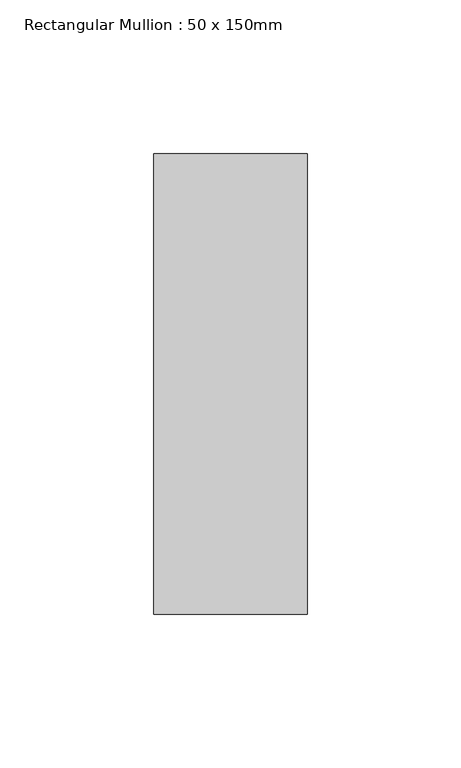
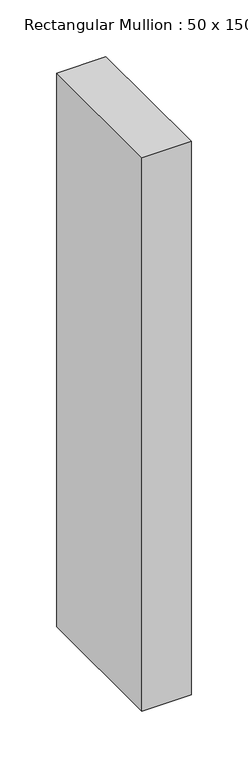
"""IFC4 building model written with IfcOpenShell, lengths in millimetres: member geometry, Rectangular Mullion : 50 x 150mm."""

import ifcopenshell
import ifcopenshell.guid

model = None  # the IFC model being written
_history = None  # IfcOwnerHistory: only IFC2X3 demands one
_inside = {}  # id of a spatial element -> (the spatial element, [elements in it])
_under = {}  # id of a project, library or spatial element -> (it, [spatial elements below it])
_declared = {}  # id of a project -> (the project, [libraries it declares])
_typed = {}  # id of a type object -> (the type object, [elements of that type])
_made_of = {}  # id of a material, layer set ... -> (it, [elements and type objects made of it])


def new_model(schema):
    """Start an empty IFC model of exactly this schema.

    Asked for "IFC4X3", IfcOpenShell would pick the latest addendum, in which some entities
    have other attributes; the version numbers below select the first issue.
    IFC2X3 requires an IfcOwnerHistory on every rooted entity: one is made here for all.
    """
    global model, _history
    if schema == "IFC4X3":
        model = ifcopenshell.file(schema_version=(4, 3, 0, 0))
    else:
        model = ifcopenshell.file(schema=schema)
    _inside.clear()
    _under.clear()
    _declared.clear()
    _typed.clear()
    _made_of.clear()
    _history = None
    if model.schema == "IFC2X3":
        org = make("IfcOrganization", Name="unknown")
        user = make(
            "IfcPersonAndOrganization",
            ThePerson=make("IfcPerson", FamilyName="unknown"),
            TheOrganization=org,
        )
        app = make(
            "IfcApplication",
            ApplicationDeveloper=org,
            Version="unknown",
            ApplicationFullName="unknown",
            ApplicationIdentifier="unknown",
        )
        _history = make(
            "IfcOwnerHistory",
            OwningUser=user,
            OwningApplication=app,
            ChangeAction="ADDED",
            CreationDate=0,
        )
    return model


def make(cls, **values):
    """One entity of the class cls with the attributes given. An attribute that is None is left unset."""
    return model.create_entity(
        cls, **{name: value for name, value in values.items() if value is not None}
    )


def rooted(cls, **values):
    """An entity with a GlobalId (a new one), such as an element, a storey or a relation."""
    return make(cls, GlobalId=ifcopenshell.guid.new(), OwnerHistory=_history, **values)


def si_unit(unit_type, name, prefix=None):
    """IfcSIUnit, for example si_unit("LENGTHUNIT", "METRE", prefix="MILLI")."""
    return make("IfcSIUnit", UnitType=unit_type, Prefix=prefix, Name=name)


def assignment(units):
    """IfcUnitAssignment: the units of a project."""
    return None if units is None else make("IfcUnitAssignment", Units=units)


def point(xyz):
    """IfcCartesianPoint."""
    return None if xyz is None else make("IfcCartesianPoint", Coordinates=xyz)


def direction(xyz):
    """IfcDirection."""
    return None if xyz is None else make("IfcDirection", DirectionRatios=xyz)


def frame(location, z_axis=None, x_axis=None):
    """IfcAxis2Placement3D, a coordinate frame: its origin and axes. An axis left out is left unset."""
    return make(
        "IfcAxis2Placement3D",
        Location=point(location),
        Axis=direction(z_axis),
        RefDirection=direction(x_axis),
    )


def origin():
    """The frame at (0, 0, 0) with its axes left unset."""
    return frame((0.0, 0.0, 0.0))


def place(relative_to, where):
    """IfcLocalPlacement: puts the frame where relative to a parent placement (None: the world)."""
    return make(
        "IfcLocalPlacement", PlacementRelTo=relative_to, RelativePlacement=where
    )


def context(
    kind, dimensions, precision=None, world=None, true_north=None, identifier=None
):
    """IfcGeometricRepresentationContext, for example the 3D "Model" context."""
    return make(
        "IfcGeometricRepresentationContext",
        ContextIdentifier=identifier,
        ContextType=kind,
        CoordinateSpaceDimension=dimensions,
        Precision=precision,
        WorldCoordinateSystem=world,
        TrueNorth=true_north,
    )


def project(units=None, contexts=None):
    """IfcProject with its units and contexts."""
    return rooted(
        "IfcProject",
        Name="project",
        RepresentationContexts=contexts,
        UnitsInContext=assignment(units),
    )


def spatial(cls, under=None, at=None, **own):
    """A site, building, storey or space (cls), placed at a placement, below another one or the project."""
    s = rooted(cls, ObjectPlacement=at, **own)
    if under is not None:
        _under.setdefault(under.id(), (under, []))[1].append(s)
    return s


def polyline(points):
    """IfcPolyline through the points."""
    return make("IfcPolyline", Points=[point(p) for p in points])


def outline(outer, holes=None, kind="AREA"):
    """IfcArbitraryClosedProfileDef: a profile drawn as a closed curve; with holes, ...WithVoids."""
    if holes is None:
        return make("IfcArbitraryClosedProfileDef", ProfileType=kind, OuterCurve=outer)
    return make(
        "IfcArbitraryProfileDefWithVoids",
        ProfileType=kind,
        OuterCurve=outer,
        InnerCurves=holes,
    )


def extrude(swept, where, along, depth):
    """IfcExtrudedAreaSolid: the profile swept, set in the frame where, extruded along a direction by depth."""
    return make(
        "IfcExtrudedAreaSolid",
        SweptArea=swept,
        Position=where,
        ExtrudedDirection=direction(along),
        Depth=depth,
    )


def shape(context_of_items, identifier, shape_type, items):
    """IfcShapeRepresentation: the items that make up one representation, for example the "Body"."""
    return make(
        "IfcShapeRepresentation",
        ContextOfItems=context_of_items,
        RepresentationIdentifier=identifier,
        RepresentationType=shape_type,
        Items=items,
    )


def source(mapping_origin, context_of_items, identifier, shape_type, items):
    """IfcRepresentationMap: a shape defined once, which mapped items show again and again."""
    return make(
        "IfcRepresentationMap",
        MappingOrigin=mapping_origin,
        MappedRepresentation=shape(context_of_items, identifier, shape_type, items),
    )


def transform(
    local_origin,
    x_axis=None,
    y_axis=None,
    z_axis=None,
    scale=None,
    scale2=None,
    scale3=None,
    uniform=True,
):
    """IfcCartesianTransformationOperator3D, or its non-uniform kind. x_axis, y_axis, z_axis: its Axis1, 2, 3."""
    if uniform:
        return make(
            "IfcCartesianTransformationOperator3D",
            Axis1=direction(x_axis),
            Axis2=direction(y_axis),
            LocalOrigin=point(local_origin),
            Scale=scale,
            Axis3=direction(z_axis),
        )
    return make(
        "IfcCartesianTransformationOperator3DnonUniform",
        Axis1=direction(x_axis),
        Axis2=direction(y_axis),
        LocalOrigin=point(local_origin),
        Scale=scale,
        Axis3=direction(z_axis),
        Scale2=scale2,
        Scale3=scale3,
    )


def mapped(mapping_source, mapping_target):
    """IfcMappedItem: shows the shape of a source again, moved by a transform."""
    return make(
        "IfcMappedItem", MappingSource=mapping_source, MappingTarget=mapping_target
    )


def made_of(thing, what):
    """Note that an element or type object is made of a material, layer set ...; save() writes the relation."""
    if what is not None:
        _made_of.setdefault(what.id(), (what, []))[1].append(thing)
    return thing


def element(
    cls,
    number,
    at=None,
    inside=None,
    cuts=None,
    type_object=None,
    material=None,
    context=None,
    identifier="Body",
    shape_type=None,
    held_by="IfcProductDefinitionShape",
    body=None,
    shapes=None,
    **own,
):
    """One element of the class cls, such as IfcWall. Its Tag is "e" and its number.

    at: its placement. inside: the storey or other place that contains it. cuts: it is an
    opening in that element (IfcRelVoidsElement). A single representation is given by context,
    identifier, shape_type and body (its items); several are given by shapes. held_by: the class
    of the entity that holds the representations. save() writes the other relations.
    """
    e = rooted(cls, Tag="e%d" % number, ObjectPlacement=at, **own)
    if body is not None:
        shapes = [shape(context, identifier, shape_type, body)]
    if shapes is not None:
        e.Representation = make(held_by, Representations=shapes)
    if inside is not None:
        _inside.setdefault(inside.id(), (inside, []))[1].append(e)
    if cuts is not None:
        rooted(
            "IfcRelVoidsElement", RelatingBuildingElement=cuts, RelatedOpeningElement=e
        )
    if type_object is not None:
        _typed.setdefault(type_object.id(), (type_object, []))[1].append(e)
    return made_of(e, material)


def aggregate(whole, parts):
    """IfcRelAggregates: a whole, such as a stair, and the parts it consists of."""
    return rooted("IfcRelAggregates", RelatingObject=whole, RelatedObjects=parts)


def save(model, path):
    """Write the relations noted so far, then the file.

    IfcRelAggregates (storeys below a building ...), IfcRelContainedInSpatialStructure (elements
    in a storey), IfcRelDefinesByType, IfcRelAssociatesMaterial and IfcRelDeclares: one each for
    every whole, place, type object, material and project.
    """
    for whole, parts in _under.values():
        aggregate(whole, parts)
    for where, things in _inside.values():
        rooted(
            "IfcRelContainedInSpatialStructure",
            RelatedElements=things,
            RelatingStructure=where,
        )
    for kind, things in _typed.values():
        rooted("IfcRelDefinesByType", RelatedObjects=things, RelatingType=kind)
    for what, things in _made_of.values():
        rooted("IfcRelAssociatesMaterial", RelatedObjects=things, RelatingMaterial=what)
    for by, libraries in _declared.values():
        rooted("IfcRelDeclares", RelatingContext=by, RelatedDefinitions=libraries)
    model.write(path)


def rectangular_mullion_50_x_150mm_431ffd9c(model_context):
    return source(origin(), model_context, "Body", "SweptSolid", [
        extrude(outline(polyline([(25.0, 75.0), (25.0, -75.0), (-25.0, -75.0), (-25.0, 75.0), (25.0, 75.0)])), frame((0.0, 0.0, -595.0), z_axis=(0.0, 0.0, 1.0), x_axis=(1.0, 0.0, 0.0)), (0.0, 0.0, 1.0), 595.0),
    ])


if __name__ == "__main__":
    model = new_model("IFC4")
    model_context = context("Model", 3, world=origin())
    ifc_project = project(units=[si_unit("LENGTHUNIT", "METRE", prefix="MILLI")], contexts=[model_context])
    site = spatial("IfcSite", under=ifc_project)
    building = spatial("IfcBuilding", under=site)
    placement = place(None, origin())
    rectangular_mullion_50_x_150mm_shape = rectangular_mullion_50_x_150mm_431ffd9c(model_context)
    element("IfcMember", 1, ObjectType="Rectangular Mullion : 50 x 150mm", at=placement, inside=building, context=model_context, shape_type="MappedRepresentation", body=[
        mapped(rectangular_mullion_50_x_150mm_shape, transform((0.0, 0.0, 0.0), x_axis=(1.0, 0.0, 0.0), y_axis=(0.0, 1.0, 0.0), z_axis=(0.0, 0.0, 1.0))),
    ])
    save(model, "model.ifc")

# Revit data of these elements
# Type "Rectangular Mullion : 50 x 150mm"
#   built-in parameter 1007304 = 0.492126 (stored number, unit not read)
#   built-in parameter 1007301 = 0.082021 (stored number, unit not read)
#   built-in parameter 1007300 = 0.082021 (stored number, unit not read)
# Element 1 (IfcMember, "Rectangular Mullion : 50 x 150mm")
#   Materials on its faces: "Metal - Aluminium"
# Materials
#   "Metal - Aluminium": class "Metal", colour RGB 247 247 247, transparency 0
